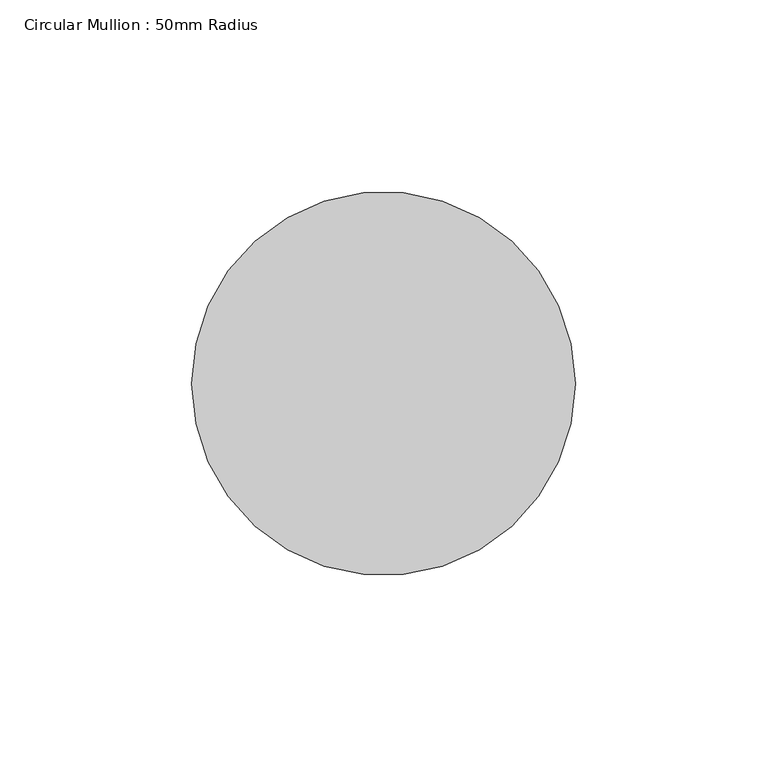
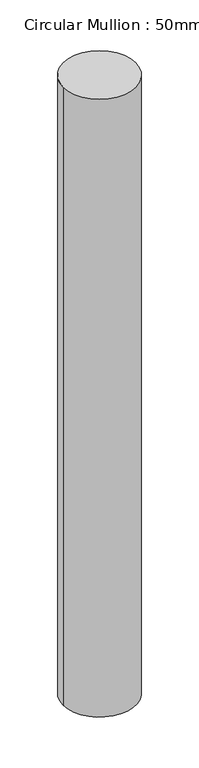
"""IFC4 building model written with IfcOpenShell, lengths in millimetres: member geometry, Circular Mullion : 50mm Radius."""

from ifc_helpers import new_model, si_unit, point, frame, origin, origin_2d, place, context, project, spatial, circle_curve, trimmed, segment, composite_curve, outline, extrude, source, transform, mapped, element, save


def circular_mullion_50mm_radius_fa43f01a(model_context):
    return source(origin(), model_context, "Body", "SweptSolid", [
        extrude(outline(composite_curve([segment(trimmed(circle_curve(origin_2d(), 50.0), [point((50.0, 0.0))], [point((-50.0, 0.0))], False, "CARTESIAN"), True, "CONTINUOUS"), segment(trimmed(circle_curve(origin_2d(), 50.0), [point((-50.0, 0.0))], [point((50.0, 0.0))], False, "CARTESIAN"), True, "CONTINUOUS")], self_intersect=False)), frame((0.0, 0.0, -897.0845576), z_axis=(0.0, 0.0, 1.0), x_axis=(1.0, 0.0, 0.0)), (0.0, 0.0, 1.0), 897.0845576),
    ])


if __name__ == "__main__":
    model = new_model("IFC4")
    model_context = context("Model", 3, world=origin())
    ifc_project = project(units=[si_unit("LENGTHUNIT", "METRE", prefix="MILLI")], contexts=[model_context])
    site = spatial("IfcSite", under=ifc_project)
    building = spatial("IfcBuilding", under=site)
    placement = place(None, origin())
    circular_mullion_50mm_radius_shape = circular_mullion_50mm_radius_fa43f01a(model_context)
    element("IfcMember", 1, ObjectType="Circular Mullion : 50mm Radius", at=placement, inside=building, context=model_context, shape_type="MappedRepresentation", body=[
        mapped(circular_mullion_50mm_radius_shape, transform((0.0, 0.0, 0.0), x_axis=(1.0, 0.0, 0.0), y_axis=(0.0, 1.0, 0.0), z_axis=(0.0, 0.0, 1.0))),
    ])
    save(model, "model.ifc")

# Revit data of these elements
# Type "Circular Mullion : 50mm Radius"
#   built-in parameter 1007350 = 0.164042 (stored number, unit not read)
# Element 1 (IfcMember, "Circular Mullion : 50mm Radius")
#   Materials on its faces: "Aluminium"
# Materials
#   "Aluminium": class "Metal", colour RGB 247 247 247, transparency 0, Description = "Aluminium 6061", Cost = 0
